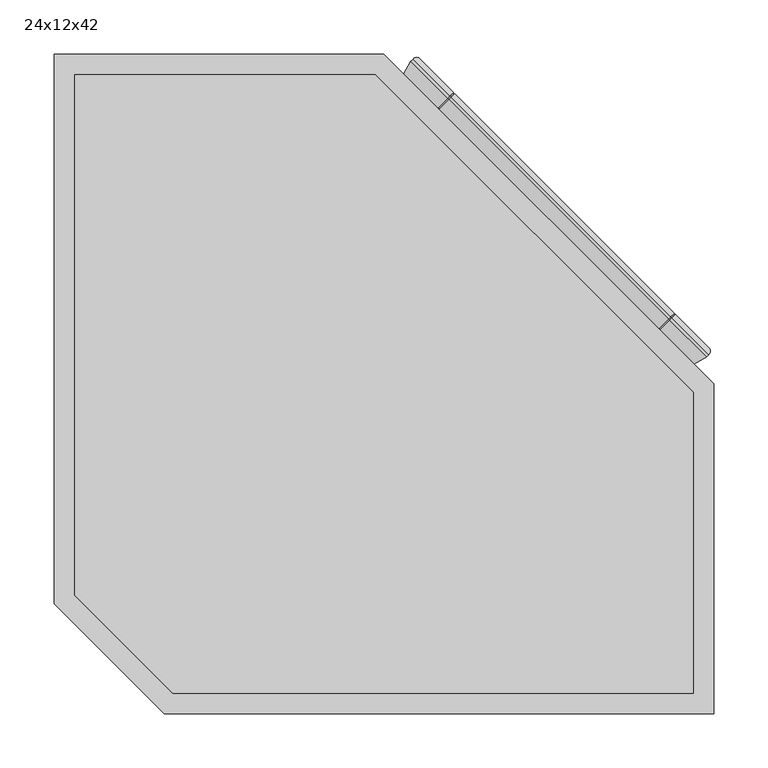
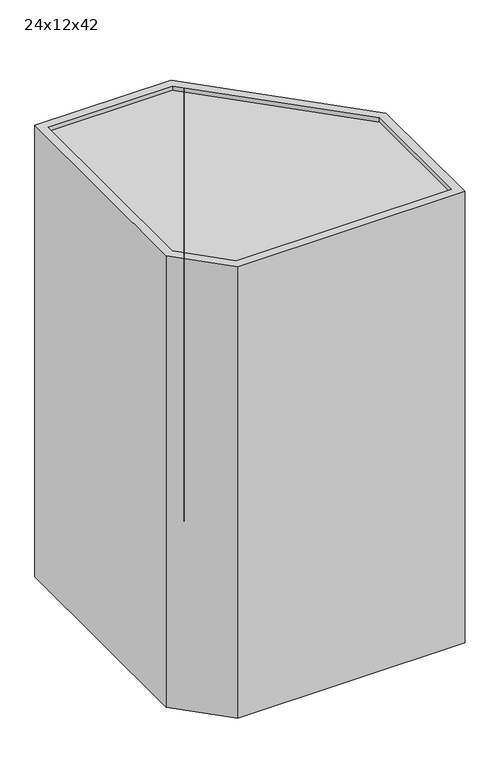
"""IFC4 building model written with IfcOpenShell, lengths in millimetres: furniture geometry, Cabinet-Wall-Merillat-Angle_Single_Door-Marlin : 24x12x42."""

from ifc_helpers import new_model, si_unit, frame, origin, place, context, project, spatial, polyline, circle_curve, ellipse_curve, outline, extrude, faceted_brep, source, transform, mapped, element, save
from ifc_brep_helpers import plane_surface, cylinder_surface, advanced_brep


def furniture_24x12x42_404ecca9(model_context):
    return source(origin(), model_context, "Body", "SolidModel", [
        advanced_brep(
        [(-277.8609132, 92.3131325, 2451.1), (-272.5103122, 93.2846318, 2448.0035075), (-272.5103122, 93.2846318, 1438.1964925), (-277.8609132, 92.3131325, 1435.1), (-279.818609, 90.3554366, 1435.1), (-279.818609, 90.3554366, 2451.1), (-286.5897222, 78.6272222, 1438.6052), (-286.5897222, 78.6272222, 2447.5948), (-254.9849038, 47.0224038, 2402.8988372), (-254.9849038, 47.0224038, 1483.3011628), (-254.1619151, 47.3219472, 1483.6712945), (-249.5344535, 49.0062055, 1485.7524535), (-249.5344535, 49.0062055, 2400.4475465), (-254.1619151, 47.3219472, 2402.5287055), (-248.9402505, 51.5799814, 1484.352684), (-248.9402505, 51.5799814, 2401.847316), (-258.8946123, 61.8880247, 1470.025), (-258.8946123, 61.8880247, 2416.175), (-255.4821149, 65.3005221, 1470.025), (-255.4821149, 65.3005221, 2416.175), (-245.1740716, 55.3461603, 1484.352684), (-245.1740716, 55.3461603, 2401.847316), (-242.6002957, 55.9403633, 1485.7524535), (-242.6002957, 55.9403633, 2400.4475465), (-240.9160374, 60.5678249, 1483.6712945), (-240.6188146, 61.3844378, 1483.3040302), (-240.616494, 61.3908136, 2402.8988372), (-240.9160374, 60.5678249, 2402.5287055), (-240.6144664, 61.388786, 1438.1964925), (-243.7755166, 58.2277358, 1435.1), (-3.5528682, -175.6728122, 1438.1964925), (-4.5243675, -181.0234132, 1435.1), (-38.5816131, -146.9661676, 1435.1), (-35.420563, -143.8051174, 1438.1964925), (-242.6529845, 57.1052038, 1435.1), (-239.4919344, 60.266254, 1438.1964925), (-36.543095, -142.6825854, 1438.1964925), (-39.7041452, -145.8436356, 1435.1), (-245.7332124, 56.27004, 1435.1), (-6.4820634, -182.981109, 1435.1), (-40.539309, -148.9238634, 1435.1), (-244.6106804, 55.147508, 1435.1), (-41.661841, -147.8013314, 1435.1), (-254.9828762, 47.0203762, 1438.6052), (-18.2102778, -189.7522222, 1438.6052), (-49.7889728, -158.1735272, 1438.6052), (-253.8603442, 45.8978442, 1438.6052), (-50.9115048, -157.0509952, 1438.6052), (-47.8312945, -152.6969535, 1485.7524535), (-253.2990782, 46.4591102, 1483.6712945), (-253.8603442, 45.8978442, 1483.3011628), (-50.9115048, -157.0509952, 1483.3011628), (-50.3502388, -156.4897292, 1483.6712945), (-49.5155528, -157.3244151, 1483.6712945), (-45.2575186, -152.1027505, 1484.352684), (-34.9494753, -162.0571123, 1470.025), (-31.5369779, -158.6446149, 1470.025), (-41.4913397, -148.3365716, 1484.352684), (-40.8971367, -145.7627957, 1485.7524535), (-36.2696751, -144.0785374, 1483.6712945), (-37.104361, -143.2438514, 1483.6712945), (-36.543095, -142.6825854, 1483.3011628), (-239.4919344, 60.266254, 1483.3011628), (-240.0532004, 59.704988, 1483.6712945), (-3.5528682, -175.6728122, 2448.0035075), (-4.5243675, -181.0234132, 2451.1), (-6.4820634, -182.981109, 2451.1), (-18.2102778, -189.7522222, 2447.5948), (-49.8150962, -158.1474038, 1483.3011628), (-49.8150962, -158.1474038, 2402.8988372), (-49.5155528, -157.3244151, 2402.5287055), (-47.8312945, -152.6969535, 2400.4475465), (-45.2575186, -152.1027505, 2401.847316), (-34.9494753, -162.0571123, 2416.175), (-31.5369779, -158.6446149, 2416.175), (-41.4913397, -148.3365716, 2401.847316), (-40.8971367, -145.7627957, 2400.4475465), (-36.2696751, -144.0785374, 2402.5287055), (-35.4466864, -143.778994, 2402.8988372), (-35.4466864, -143.778994, 1483.3011628), (-35.420563, -143.8051174, 2448.0035075), (-38.5816131, -146.9661676, 2451.1), (-243.7755166, 58.2277358, 2451.1), (-240.6144664, 61.388786, 2448.0035075), (-39.7041452, -145.8436356, 2451.1), (-36.543095, -142.6825854, 2448.0035075), (-239.4919344, 60.266254, 2448.0035075), (-242.6529845, 57.1052038, 2451.1), (-40.539309, -148.9238634, 2451.1), (-245.7332124, 56.27004, 2451.1), (-41.661841, -147.8013314, 2451.1), (-244.6106804, 55.147508, 2451.1), (-49.7889728, -158.1735272, 2447.5948), (-254.9828762, 47.0203762, 2447.5948), (-50.9115048, -157.0509952, 2447.5948), (-253.8603442, 45.8978442, 2447.5948), (-50.9115048, -157.0509952, 2402.8988372), (-253.8603442, 45.8978442, 2402.8988372), (-50.3502388, -156.4897292, 2402.5287055), (-253.2990782, 46.4591102, 2402.5287055), (-240.0532004, 59.704988, 2402.5287055), (-239.4919344, 60.266254, 2402.8988372), (-36.543095, -142.6825854, 2402.8988372), (-37.104361, -143.2438514, 2402.5287055), (-50.3502388, -156.4897292, 2446.9857412), (-41.5879457, -147.7274361, 2450.30625), (-39.7041452, -145.8436356, 2450.30625), (-37.104361, -143.2438514, 2447.8526052), (-35.981829, -144.3663834, 2402.5287055), (-35.981829, -144.3663834, 2447.8526052), (-38.5816131, -146.9661676, 2450.30625), (-40.4654137, -148.8499682, 2450.30625), (-49.2277068, -157.6122612, 2446.9857412), (-49.2277068, -157.6122612, 2402.5287055), (-254.4216102, 47.5816422, 2402.5287055), (-254.4216102, 47.5816422, 2446.9857412), (-245.6593171, 56.3439353, 2450.30625), (-243.7755166, 58.2277358, 2450.30625), (-241.1757324, 60.82752, 2447.8526052), (-241.1757324, 60.82752, 2402.5287055), (-240.0532004, 59.704988, 2447.8526052), (-242.6529845, 57.1052038, 2450.30625), (-244.5367851, 55.2214033, 2450.30625), (-253.2990782, 46.4591102, 2446.9857412), (-241.1757324, 60.82752, 1483.6712945), (-241.1757324, 60.82752, 1438.3473948), (-243.7755166, 58.2277358, 1435.89375), (-245.6593171, 56.3439353, 1435.89375), (-254.4216102, 47.5816422, 1439.2142588), (-254.4216102, 47.5816422, 1483.6712945), (-253.2990782, 46.4591102, 1439.2142588), (-244.5367851, 55.2214033, 1435.89375), (-242.6529845, 57.1052038, 1435.89375), (-240.0532004, 59.704988, 1438.3473948), (-37.104361, -143.2438514, 1438.3473948), (-39.7041452, -145.8436356, 1435.89375), (-41.5879457, -147.7274361, 1435.89375), (-50.3502388, -156.4897292, 1439.2142588), (-35.981829, -144.3663834, 1483.6712945), (-49.2277068, -157.6122612, 1483.6712945), (-49.2277068, -157.6122612, 1439.2142588), (-40.4654137, -148.8499682, 1435.89375), (-38.5816131, -146.9661676, 1435.89375), (-35.981829, -144.3663834, 1438.3473948)],
        [
            (0, 1, ellipse_curve(frame((-274.4843369, 88.9365562, 2446.3248), z_axis=(-0.5000000000000046, 0.49999999999999534, -0.7071067811865475), x_axis=(-0.5000000000000044, 0.4999999999999953, 0.7071067811865476)), 6.7531526, 4.7752)),
            (1, 2),
            (2, 3, ellipse_curve(frame((-274.4843369, 88.9365562, 1439.8752), z_axis=(-0.5000000000000046, 0.49999999999999534, 0.7071067811865475), x_axis=(0.5000000000000044, -0.4999999999999953, 0.7071067811865476)), 6.7531526, 4.7752)),
            (3, 0),
            (3, 4),
            (4, 5),
            (5, 0),
            (4, 6),
            (6, 7),
            (7, 5),
            (8, 9),
            (9, 10),
            (10, 11),
            (11, 12),
            (12, 13),
            (13, 8),
            (11, 14, ellipse_curve(frame((-250.0730668, 50.4860334, 1484.3252), z_axis=(-0.5000000000000047, 0.49999999999999545, 0.7071067811865475), x_axis=(0.5000000000000046, -0.49999999999999534, 0.7071067811865476)), 2.2271035, 1.5748)),
            (14, 15),
            (15, 12, ellipse_curve(frame((-250.0730668, 50.4860334, 2401.8748), z_axis=(-0.5000000000000047, 0.49999999999999545, -0.7071067811865475), x_axis=(-0.5000000000000046, 0.49999999999999534, 0.7071067811865476)), 2.2271035, 1.5748)),
            (14, 16),
            (16, 17),
            (17, 15),
            (16, 18),
            (18, 19),
            (19, 17),
            (18, 20),
            (20, 21),
            (21, 19),
            (20, 22, ellipse_curve(frame((-244.0801236, 56.4789766, 1484.3252), z_axis=(-0.5000000000000047, 0.49999999999999545, 0.7071067811865475), x_axis=(0.5000000000000046, -0.49999999999999534, 0.7071067811865476)), 2.2271035, 1.5748)),
            (22, 23),
            (23, 21, ellipse_curve(frame((-244.0801236, 56.4789766, 2401.8748), z_axis=(-0.5000000000000047, 0.49999999999999545, -0.7071067811865475), x_axis=(-0.5000000000000046, 0.49999999999999534, 0.7071067811865476)), 2.2271035, 1.5748)),
            (22, 24),
            (24, 25),
            (25, 26),
            (26, 27),
            (27, 23),
            (2, 28),
            (28, 29, circle_curve(frame((-243.7755166, 58.2277358, 1439.8752), z_axis=(-0.707106781186554, 0.707106781186541, 0.0), x_axis=(-0.707106781186541, -0.707106781186554, 0.0)), 4.7752)),
            (29, 3),
            (30, 31, ellipse_curve(frame((-7.9009438, -177.6468369, 1439.8752), z_axis=(-0.5000000000000046, 0.49999999999999534, -0.7071067811865475), x_axis=(-0.5000000000000047, 0.4999999999999955, 0.7071067811865475)), 6.7531526, 4.7752)),
            (31, 32),
            (32, 33, circle_curve(frame((-38.5816131, -146.9661676, 1439.8752), z_axis=(0.707106781186554, -0.707106781186541, 0.0), x_axis=(-0.707106781186541, -0.707106781186554, 0.0)), 4.7752)),
            (33, 30),
            (34, 35, circle_curve(frame((-242.6529845, 57.1052038, 1439.8752), z_axis=(0.707106781186554, -0.707106781186541, 0.0), x_axis=(-0.707106781186541, -0.707106781186554, 0.0)), 4.7752)),
            (35, 36),
            (36, 37, circle_curve(frame((-39.7041452, -145.8436356, 1439.8752), z_axis=(-0.707106781186554, 0.707106781186541, 0.0), x_axis=(-0.707106781186541, -0.707106781186554, 0.0)), 4.7752)),
            (37, 34),
            (29, 38),
            (38, 4),
            (31, 39),
            (39, 40),
            (40, 32),
            (41, 34),
            (37, 42),
            (42, 41),
            (38, 43),
            (43, 6),
            (39, 44),
            (44, 45),
            (45, 40),
            (46, 41),
            (42, 47),
            (47, 46),
            (48, 11),
            (10, 49),
            (49, 50),
            (50, 51),
            (51, 52),
            (52, 53),
            (53, 48),
            (48, 54, ellipse_curve(frame((-46.3514666, -153.2355668, 1484.3252), z_axis=(-0.5000000000000047, 0.49999999999999545, -0.7071067811865475), x_axis=(-0.5000000000000046, 0.49999999999999534, 0.7071067811865476)), 2.2271035, 1.5748)),
            (54, 14),
            (54, 55),
            (55, 16),
            (55, 56),
            (56, 18),
            (56, 57),
            (57, 20),
            (57, 58, ellipse_curve(frame((-40.3585234, -147.2426236, 1484.3252), z_axis=(-0.5000000000000047, 0.49999999999999545, -0.7071067811865475), x_axis=(-0.5000000000000046, 0.49999999999999534, 0.7071067811865476)), 2.2271035, 1.5748)),
            (58, 22),
            (58, 59),
            (59, 60),
            (60, 61),
            (61, 62),
            (62, 63),
            (63, 24),
            (30, 64),
            (64, 65, ellipse_curve(frame((-7.9009438, -177.6468369, 2446.3248), z_axis=(0.5000000000000046, -0.49999999999999534, -0.7071067811865475), x_axis=(-0.5000000000000044, 0.4999999999999953, -0.7071067811865476)), 6.7531526, 4.7752)),
            (65, 31),
            (65, 66),
            (66, 39),
            (66, 67),
            (67, 44),
            (68, 69),
            (69, 70),
            (70, 71),
            (71, 48),
            (53, 68),
            (71, 72, ellipse_curve(frame((-46.3514666, -153.2355668, 2401.8748), z_axis=(0.5000000000000047, -0.49999999999999545, -0.7071067811865475), x_axis=(-0.5000000000000046, 0.49999999999999534, -0.7071067811865476)), 2.2271035, 1.5748)),
            (72, 54),
            (72, 73),
            (73, 55),
            (73, 74),
            (74, 56),
            (74, 75),
            (75, 57),
            (75, 76, ellipse_curve(frame((-40.3585234, -147.2426236, 2401.8748), z_axis=(0.5000000000000047, -0.49999999999999545, -0.7071067811865475), x_axis=(-0.5000000000000046, 0.49999999999999534, -0.7071067811865476)), 2.2271035, 1.5748)),
            (76, 58),
            (76, 77),
            (77, 78),
            (78, 79),
            (79, 59),
            (64, 80),
            (80, 81, circle_curve(frame((-38.5816131, -146.9661676, 2446.3248), z_axis=(0.707106781186554, -0.707106781186541, 0.0), x_axis=(-0.707106781186541, -0.707106781186554, 0.0)), 4.7752)),
            (81, 65),
            (0, 82),
            (82, 83, circle_curve(frame((-243.7755166, 58.2277358, 2446.3248), z_axis=(-0.707106781186554, 0.707106781186541, 0.0), x_axis=(-0.707106781186541, -0.707106781186554, 0.0)), 4.7752)),
            (83, 1),
            (84, 85, circle_curve(frame((-39.7041452, -145.8436356, 2446.3248), z_axis=(-0.707106781186554, 0.707106781186541, 0.0), x_axis=(-0.707106781186541, -0.707106781186554, 0.0)), 4.7752)),
            (85, 86),
            (86, 87, circle_curve(frame((-242.6529845, 57.1052038, 2446.3248), z_axis=(0.707106781186554, -0.707106781186541, 0.0), x_axis=(-0.707106781186541, -0.707106781186554, 0.0)), 4.7752)),
            (87, 84),
            (81, 88),
            (88, 66),
            (5, 89),
            (89, 82),
            (90, 84),
            (87, 91),
            (91, 90),
            (88, 92),
            (92, 67),
            (7, 93),
            (93, 89),
            (94, 90),
            (91, 95),
            (95, 94),
            (43, 9),
            (8, 93),
            (92, 69),
            (68, 45),
            (96, 94),
            (95, 97),
            (97, 96),
            (50, 46),
            (47, 51),
            (12, 71),
            (70, 98),
            (98, 96),
            (97, 99),
            (99, 13),
            (15, 72),
            (17, 73),
            (19, 74),
            (21, 75),
            (23, 76),
            (27, 100),
            (100, 101),
            (101, 102),
            (102, 103),
            (103, 77),
            (83, 26),
            (25, 28),
            (33, 79),
            (78, 80),
            (85, 102),
            (101, 86),
            (35, 62),
            (61, 36),
            (98, 104),
            (104, 105),
            (105, 106),
            (106, 107, circle_curve(frame((-39.7041452, -145.8436356, 2446.3248), z_axis=(-0.7071067811865612, 0.7071067811865338, 0.0), x_axis=(0.0, 0.0, 1.0)), 3.98145)),
            (107, 103),
            (78, 108),
            (108, 109),
            (109, 110, circle_curve(frame((-38.5816131, -146.9661676, 2446.3248), z_axis=(0.7071067811865612, -0.7071067811865338, 0.0), x_axis=(0.0, 0.0, 1.0)), 3.98145)),
            (110, 111),
            (111, 112),
            (112, 113),
            (113, 69),
            (77, 108),
            (107, 109),
            (106, 110),
            (105, 111),
            (104, 112),
            (70, 113),
            (8, 114),
            (114, 115),
            (115, 116),
            (116, 117),
            (117, 118, circle_curve(frame((-243.7755166, 58.2277358, 2446.3248), z_axis=(-0.7071067811865612, 0.7071067811865338, 0.0), x_axis=(0.0, 0.0, 1.0)), 3.98145)),
            (118, 119),
            (119, 26),
            (100, 120),
            (120, 121, circle_curve(frame((-242.6529845, 57.1052038, 2446.3248), z_axis=(0.7071067811865612, -0.7071067811865338, 0.0), x_axis=(0.0, 0.0, 1.0)), 3.98145)),
            (121, 122),
            (122, 123),
            (123, 99),
            (119, 27),
            (118, 120),
            (117, 121),
            (116, 122),
            (115, 123),
            (114, 13),
            (25, 124),
            (124, 125),
            (125, 126, circle_curve(frame((-243.7755166, 58.2277358, 1439.8752), z_axis=(-0.7071067811865612, 0.7071067811865338, 0.0), x_axis=(0.0, 0.0, 1.0)), 3.98145)),
            (126, 127),
            (127, 128),
            (128, 129),
            (129, 9),
            (49, 130),
            (130, 131),
            (131, 132),
            (132, 133, circle_curve(frame((-242.6529845, 57.1052038, 1439.8752), z_axis=(0.7071067811865612, -0.7071067811865338, 0.0), x_axis=(0.0, 0.0, 1.0)), 3.98145)),
            (133, 63),
            (129, 10),
            (128, 130),
            (127, 131),
            (126, 132),
            (125, 133),
            (124, 24),
            (60, 134),
            (134, 135, circle_curve(frame((-39.7041452, -145.8436356, 1439.8752), z_axis=(-0.7071067811865612, 0.7071067811865338, 0.0), x_axis=(0.0, 0.0, 1.0)), 3.98145)),
            (135, 136),
            (136, 137),
            (137, 52),
            (138, 79),
            (68, 139),
            (139, 140),
            (140, 141),
            (141, 142),
            (142, 143, circle_curve(frame((-38.5816131, -146.9661676, 1439.8752), z_axis=(0.7071067811865612, -0.7071067811865338, 0.0), x_axis=(0.0, 0.0, 1.0)), 3.98145)),
            (143, 138),
            (138, 59),
            (53, 139),
            (137, 140),
            (136, 141),
            (135, 142),
            (134, 143),
        ],
        [
            cylinder_surface(frame((-274.4843369, 88.9365562, 2451.1), z_axis=(0.0, 0.0, 1.0), x_axis=(-0.7071067811865398, -0.7071067811865552, 0.0)), 4.7752),
            plane_surface(frame((-277.8609132, 92.3131325, 2451.1), z_axis=(-0.7071067811865552, 0.7071067811865398, 0.0), x_axis=(0.0, 0.0, -1.0))),
            plane_surface(frame((-279.818609, 90.3554366, 2451.1), z_axis=(-0.8660309890157606, 0.49999032597079685, 0.0), x_axis=(0.0, 0.0, -1.0))),
            plane_surface(frame((-254.9849038, 47.0224038, 2402.8988372), z_axis=(0.3420201433255881, -0.9396926207859378, 0.0), x_axis=(0.0, 0.0, -1.0))),
            cylinder_surface(frame((-250.0730668, 50.4860334, 2451.1), z_axis=(0.0, 0.0, 1.0000000000000002), x_axis=(0.7193398003386519, 0.6946583704589966, 0.0)), 1.5748),
            plane_surface(frame((-248.9402505, 51.5799814, 2401.847316), z_axis=(0.7193398003386716, 0.6946583704589762, 0.0), x_axis=(0.0, 0.0, -1.0))),
            plane_surface(frame((-258.8946123, 61.8880247, 2416.175), z_axis=(0.7071067811865552, -0.7071067811865398, 0.0), x_axis=(0.0, 0.0, -1.0))),
            plane_surface(frame((-255.4821149, 65.3005221, 2416.175), z_axis=(-0.6946583704589944, -0.7193398003386541, 0.0), x_axis=(0.0, 0.0, -1.0))),
            cylinder_surface(frame((-244.0801236, 56.4789766, 2451.1), z_axis=(0.0, 0.0, 1.0000000000000002), x_axis=(0.9396926207858448, -0.3420201433258438, 0.0)), 1.5748),
            plane_surface(frame((-242.6002957, 55.9403633, 2400.4475465), z_axis=(0.9396926207859251, -0.342020143325623, 0.0), x_axis=(0.0, 0.0, -1.0))),
            cylinder_surface(frame((-277.8609132, 92.3131325, 1439.8752), z_axis=(-0.707106781186554, 0.707106781186541, 0.0), x_axis=(-0.707106781186541, -0.707106781186554, 0.0)), 4.7752),
            plane_surface(frame((-277.8609132, 92.3131325, 1435.1), z_axis=(0.0, 0.0, -1.0), x_axis=(0.707106781186554, -0.707106781186541, 0.0))),
            plane_surface(frame((-279.818609, 90.3554366, 1435.1), z_axis=(-0.18302033152247393, -0.1830203315224773, -0.9659229350723619), x_axis=(0.707106781186554, -0.707106781186541, 0.0))),
            plane_surface(frame((-254.9849038, 47.0224038, 1483.3011628), z_axis=(-0.298836238730178, -0.2988362387301835, 0.9063077870366099), x_axis=(0.707106781186554, -0.707106781186541, 0.0))),
            cylinder_surface(frame((-284.8805396, 85.2935061, 1484.3252), z_axis=(-0.7071067811865541, 0.7071067811865411, 0.0), x_axis=(0.7069990853988176, 0.7069990853988306, 0.01745240643729364)), 1.5748),
            plane_surface(frame((-248.9402505, 51.5799814, 1484.352684), z_axis=(0.7069990853988173, 0.7069990853988303, 0.017452406437322147), x_axis=(0.707106781186554, -0.707106781186541, 0.0))),
            plane_surface(frame((-258.8946123, 61.8880247, 1470.025), z_axis=(0.0, 0.0, 1.0), x_axis=(0.707106781186554, -0.707106781186541, 0.0))),
            plane_surface(frame((-255.4821149, 65.3005221, 1470.025), z_axis=(-0.7069990853988178, -0.7069990853988308, 0.01745240643727848), x_axis=(0.707106781186554, -0.707106781186541, 0.0))),
            cylinder_surface(frame((-278.8875963, 91.2864494, 1484.3252), z_axis=(-0.7071067811865541, 0.7071067811865411, 0.0), x_axis=(0.2988362387299919, 0.29883623872999737, 0.9063077870367326)), 1.5748),
            plane_surface(frame((-242.6002957, 55.9403633, 1485.7524535), z_axis=(0.29883623873014237, 0.29883623873014786, 0.9063077870366333), x_axis=(0.707106781186554, -0.707106781186541, 0.0))),
            cylinder_surface(frame((-7.9009438, -177.6468369, 1435.1), z_axis=(0.0, 0.0, -1.0), x_axis=(-0.7071067811865422, -0.7071067811865528, 0.0)), 4.7752),
            plane_surface(frame((-4.5243675, -181.0234132, 1435.1), z_axis=(0.7071067811865528, -0.7071067811865422, 0.0), x_axis=(0.0, 0.0, 1.0))),
            plane_surface(frame((-6.4820634, -182.981109, 1435.1), z_axis=(0.4999903259708127, -0.8660309890157514, 0.0), x_axis=(0.0, 0.0, 1.0))),
            plane_surface(frame((-49.8150962, -158.1474038, 1483.3011628), z_axis=(-0.939692620785944, 0.3420201433255708, 0.0), x_axis=(0.0, 0.0, 1.0))),
            cylinder_surface(frame((-46.3514666, -153.2355668, 1435.1), z_axis=(0.0, 0.0, -1.0000000000000002), x_axis=(0.6946583704589834, 0.7193398003386646, 0.0)), 1.5748),
            plane_surface(frame((-45.2575186, -152.1027505, 1484.352684), z_axis=(0.694658370458963, 0.7193398003386844, 0.0), x_axis=(0.0, 0.0, 1.0))),
            plane_surface(frame((-34.9494753, -162.0571123, 1470.025), z_axis=(-0.7071067811865528, 0.7071067811865422, 0.0), x_axis=(0.0, 0.0, 1.0))),
            plane_surface(frame((-31.5369779, -158.6446149, 1470.025), z_axis=(-0.7193398003386413, -0.6946583704590076, 0.0), x_axis=(0.0, 0.0, 1.0))),
            cylinder_surface(frame((-40.3585234, -147.2426236, 1435.1), z_axis=(0.0, 0.0, -1.0000000000000002), x_axis=(-0.34202014332586106, 0.9396926207858385, 0.0)), 1.5748),
            plane_surface(frame((-40.8971367, -145.7627957, 1485.7524535), z_axis=(-0.3420201433256403, 0.9396926207859188, 0.0), x_axis=(0.0, 0.0, 1.0))),
            cylinder_surface(frame((-4.5243675, -181.0234132, 2446.3248), z_axis=(0.707106781186554, -0.707106781186541, 0.0), x_axis=(-0.707106781186541, -0.707106781186554, 0.0)), 4.7752),
            plane_surface(frame((-4.5243675, -181.0234132, 2451.1), z_axis=(0.0, 0.0, 1.0), x_axis=(-0.707106781186554, 0.707106781186541, 0.0))),
            plane_surface(frame((-6.4820634, -182.981109, 2451.1), z_axis=(-0.18302033152247393, -0.1830203315224773, 0.9659229350723619), x_axis=(-0.707106781186554, 0.707106781186541, 0.0))),
            plane_surface(frame((-18.2102778, -189.7522222, 2447.5948), z_axis=(-0.707106781186541, -0.707106781186554, 0.0), x_axis=(-0.707106781186554, 0.707106781186541, 0.0))),
            plane_surface(frame((-49.8150962, -158.1474038, 2402.8988372), z_axis=(-0.298836238730178, -0.2988362387301835, -0.9063077870366099), x_axis=(-0.707106781186554, 0.707106781186541, 0.0))),
            cylinder_surface(frame((-11.5439939, -188.0430396, 2401.8748), z_axis=(0.7071067811865541, -0.7071067811865411, 0.0), x_axis=(0.7069990853988176, 0.7069990853988306, -0.01745240643729364)), 1.5748),
            plane_surface(frame((-45.2575186, -152.1027505, 2401.847316), z_axis=(0.7069990853988173, 0.7069990853988303, -0.017452406437322147), x_axis=(-0.707106781186554, 0.707106781186541, 0.0))),
            plane_surface(frame((-34.9494753, -162.0571123, 2416.175), z_axis=(0.0, 0.0, -1.0), x_axis=(-0.707106781186554, 0.707106781186541, 0.0))),
            plane_surface(frame((-31.5369779, -158.6446149, 2416.175), z_axis=(-0.7069990853988178, -0.7069990853988308, -0.01745240643727848), x_axis=(-0.707106781186554, 0.707106781186541, 0.0))),
            cylinder_surface(frame((-5.5510506, -182.0500963, 2401.8748), z_axis=(0.7071067811865541, -0.7071067811865411, 0.0), x_axis=(0.2988362387299919, 0.29883623872999737, -0.9063077870367326)), 1.5748),
            plane_surface(frame((-40.8971367, -145.7627957, 2400.4475465), z_axis=(0.29883623873014237, 0.29883623873014786, -0.9063077870366333), x_axis=(-0.707106781186554, 0.707106781186541, 0.0))),
            plane_surface(frame((-35.4466864, -143.778994, 2402.8988372), z_axis=(0.707106781186541, 0.707106781186554, 0.0), x_axis=(-0.707106781186554, 0.707106781186541, 0.0))),
            plane_surface(frame((-36.543095, -142.6825854, 2402.8988372), z_axis=(0.7071067811865612, -0.7071067811865337, 0.0), x_axis=(-0.6408563820557478, -0.6408563820557727, -0.4226182617407854))),
            plane_surface(frame((-35.420563, -143.8051174, 2402.8988372), z_axis=(-0.7071067811865612, 0.7071067811865337, 0.0), x_axis=(0.6408563820557478, 0.6408563820557727, 0.4226182617407854))),
            plane_surface(frame((-36.543095, -142.6825854, 2402.8988372), z_axis=(-0.2988362387301747, -0.2988362387301865, 0.9063077870366099), x_axis=(0.7071067811865616, -0.7071067811865335, 0.0))),
            plane_surface(frame((-37.104361, -143.2438514, 2402.5287055), z_axis=(0.7071067811865335, 0.7071067811865616, 0.0), x_axis=(0.7071067811865616, -0.7071067811865335, 0.0))),
            cylinder_surface(frame((-38.5816131, -146.9661676, 2446.3248), z_axis=(0.7071067811865612, -0.7071067811865338, 0.0), x_axis=(0.0, 0.0, 1.0)), 3.98145),
            plane_surface(frame((-39.7041452, -145.8436356, 2450.30625), z_axis=(0.0, 0.0, 1.0), x_axis=(0.7071067811865616, -0.7071067811865335, 0.0))),
            plane_surface(frame((-41.5879457, -147.7274361, 2450.30625), z_axis=(-0.18302033152251398, -0.18302033152252126, 0.965922935072346), x_axis=(0.7071067811865616, -0.7071067811865335, 0.0))),
            plane_surface(frame((-50.3502388, -156.4897292, 2446.9857412), z_axis=(-0.7071067811865335, -0.7071067811865616, 0.0), x_axis=(0.7071067811865616, -0.7071067811865335, 0.0))),
            plane_surface(frame((-50.3502388, -156.4897292, 2402.5287055), z_axis=(0.29883623873019277, 0.2988362387302046, 0.906307787036598), x_axis=(0.7071067811865616, -0.7071067811865335, 0.0))),
            plane_surface(frame((-240.6144664, 61.388786, 2402.8988372), z_axis=(0.7071067811865612, -0.7071067811865337, 0.0), x_axis=(-0.6408563820557478, -0.6408563820557727, -0.4226182617407854))),
            plane_surface(frame((-239.4919344, 60.266254, 2402.8988372), z_axis=(-0.7071067811865612, 0.7071067811865337, 0.0), x_axis=(0.6408563820557478, 0.6408563820557727, 0.4226182617407854))),
            plane_surface(frame((-240.6144664, 61.388786, 2402.8988372), z_axis=(-0.2988362387301747, -0.2988362387301865, 0.9063077870366099), x_axis=(0.7071067811865616, -0.7071067811865335, 0.0))),
            plane_surface(frame((-241.1757324, 60.82752, 2402.5287055), z_axis=(0.7071067811865335, 0.7071067811865616, 0.0), x_axis=(0.7071067811865616, -0.7071067811865335, 0.0))),
            cylinder_surface(frame((-242.6529845, 57.1052038, 2446.3248), z_axis=(0.7071067811865612, -0.7071067811865338, 0.0), x_axis=(0.0, 0.0, 1.0)), 3.98145),
            plane_surface(frame((-243.7755166, 58.2277358, 2450.30625), z_axis=(0.0, 0.0, 1.0), x_axis=(0.7071067811865616, -0.7071067811865335, 0.0))),
            plane_surface(frame((-245.6593171, 56.3439353, 2450.30625), z_axis=(-0.18302033152251576, -0.18302033152252303, 0.9659229350723454), x_axis=(0.7071067811865616, -0.7071067811865335, 0.0))),
            plane_surface(frame((-254.4216102, 47.5816422, 2446.9857412), z_axis=(-0.7071067811865354, -0.7071067811865597, 0.0), x_axis=(0.7071067811865597, -0.7071067811865354, 0.0))),
            plane_surface(frame((-254.4216102, 47.5816422, 2402.5287055), z_axis=(0.29883623873019416, 0.29883623873020443, 0.9063077870365974), x_axis=(0.7071067811865597, -0.7071067811865354, 0.0))),
            plane_surface(frame((-243.7755166, 58.2277358, 1444.6504), z_axis=(0.7071067811865612, -0.7071067811865338, 0.0), x_axis=(0.7071067811865338, 0.7071067811865612, 0.0))),
            plane_surface(frame((-242.6529845, 57.1052038, 1444.6504), z_axis=(-0.7071067811865612, 0.7071067811865338, 0.0), x_axis=(-0.7071067811865338, -0.7071067811865612, 0.0))),
            plane_surface(frame((-254.9828762, 47.0203762, 1483.3011628), z_axis=(0.2988362387301807, 0.2988362387301926, -0.906307787036606), x_axis=(0.7071067811865616, -0.7071067811865335, 0.0))),
            plane_surface(frame((-254.4216102, 47.5816422, 1483.6712945), z_axis=(-0.7071067811865335, -0.7071067811865616, 0.0), x_axis=(0.7071067811865616, -0.7071067811865335, 0.0))),
            plane_surface(frame((-254.4216102, 47.5816422, 1439.2142588), z_axis=(-0.18302033152271646, -0.18302033152272373, -0.9659229350722693), x_axis=(0.7071067811865616, -0.7071067811865335, 0.0))),
            plane_surface(frame((-245.6593171, 56.3439353, 1435.89375), z_axis=(0.0, 0.0, -1.0), x_axis=(0.7071067811865616, -0.7071067811865335, 0.0))),
            cylinder_surface(frame((-242.6529845, 57.1052038, 1439.8752), z_axis=(0.7071067811865612, -0.7071067811865338, 0.0), x_axis=(0.0, 0.0, 1.0)), 3.98145),
            plane_surface(frame((-241.1757324, 60.82752, 1438.3473948), z_axis=(0.7071067811865335, 0.7071067811865616, 0.0), x_axis=(0.7071067811865616, -0.7071067811865335, 0.0))),
            plane_surface(frame((-241.1757324, 60.82752, 1483.6712945), z_axis=(-0.29883623873017934, -0.2988362387301912, -0.906307787036607), x_axis=(0.7071067811865616, -0.7071067811865335, 0.0))),
            plane_surface(frame((-37.104361, -143.2438514, 1483.6712945), z_axis=(0.7071067811865613, -0.7071067811865339, 0.0), x_axis=(0.6408563820557613, 0.6408563820557862, -0.42261826174074446))),
            plane_surface(frame((-35.981829, -144.3663834, 1483.6712945), z_axis=(-0.7071067811865613, 0.7071067811865339, 0.0), x_axis=(-0.6408563820557613, -0.6408563820557862, 0.42261826174074446))),
            plane_surface(frame((-37.104361, -143.2438514, 1483.6712945), z_axis=(-0.2988362387301457, -0.2988362387301576, -0.9063077870366291), x_axis=(0.7071067811865616, -0.7071067811865335, 0.0))),
            plane_surface(frame((-50.9115048, -157.0509952, 1483.3011628), z_axis=(0.2988362387301807, 0.2988362387301926, -0.906307787036606), x_axis=(0.7071067811865616, -0.7071067811865335, 0.0))),
            plane_surface(frame((-50.3502388, -156.4897292, 1483.6712945), z_axis=(-0.7071067811865335, -0.7071067811865616, 0.0), x_axis=(0.7071067811865616, -0.7071067811865335, 0.0))),
            plane_surface(frame((-50.3502388, -156.4897292, 1439.2142588), z_axis=(-0.1830203315227165, -0.18302033152272376, -0.9659229350722693), x_axis=(0.7071067811865616, -0.7071067811865335, 0.0))),
            plane_surface(frame((-41.5879457, -147.7274361, 1435.89375), z_axis=(0.0, 0.0, -1.0), x_axis=(0.7071067811865616, -0.7071067811865335, 0.0))),
            cylinder_surface(frame((-38.5816131, -146.9661676, 1439.8752), z_axis=(0.7071067811865612, -0.7071067811865338, 0.0), x_axis=(0.0, 0.0, 1.0)), 3.98145),
            plane_surface(frame((-37.104361, -143.2438514, 1438.3473948), z_axis=(0.7071067811865335, 0.7071067811865616, 0.0), x_axis=(0.7071067811865616, -0.7071067811865335, 0.0))),
        ],
        [
            (0, [[1, 2, 3, 4]]),
            (1, [[-4, 5, 6, 7]]),
            (2, [[-6, 8, 9, 10]]),
            (3, [[11, 12, 13, 14, 15, 16]]),
            (4, [[-14, 17, 18, 19]]),
            (5, [[-18, 20, 21, 22]]),
            (6, [[-21, 23, 24, 25]]),
            (7, [[-24, 26, 27, 28]]),
            (8, [[-27, 29, 30, 31]]),
            (9, [[-30, 32, 33, 34, 35, 36]]),
            (10, [[-3, 37, 38, 39]]),
            (10, [[40, 41, 42, 43]]),
            (10, [[44, 45, 46, 47]]),
            (11, [[-5, -39, 48, 49]]),
            (11, [[50, 51, 52, -41]]),
            (11, [[53, -47, 54, 55]]),
            (12, [[-8, -49, 56, 57]]),
            (12, [[58, 59, 60, -51]]),
            (12, [[61, -55, 62, 63]]),
            (13, [[64, -13, 65, 66, 67, 68, 69, 70]]),
            (14, [[-17, -64, 71, 72]]),
            (15, [[-20, -72, 73, 74]]),
            (16, [[-23, -74, 75, 76]]),
            (17, [[-26, -76, 77, 78]]),
            (18, [[-29, -78, 79, 80]]),
            (19, [[-80, 81, 82, 83, 84, 85, 86, -32]]),
            (20, [[-40, 87, 88, 89]]),
            (21, [[-50, -89, 90, 91]]),
            (22, [[-58, -91, 92, 93]]),
            (23, [[94, 95, 96, 97, -70, 98]]),
            (24, [[-71, -97, 99, 100]]),
            (25, [[-73, -100, 101, 102]]),
            (26, [[-75, -102, 103, 104]]),
            (27, [[-77, -104, 105, 106]]),
            (28, [[-79, -106, 107, 108]]),
            (29, [[-108, 109, 110, 111, 112, -81]]),
            (30, [[-88, 113, 114, 115]]),
            (30, [[-1, 116, 117, 118]]),
            (30, [[119, 120, 121, 122]]),
            (31, [[-90, -115, 123, 124]]),
            (31, [[-7, 125, 126, -116]]),
            (31, [[127, -122, 128, 129]]),
            (32, [[-92, -124, 130, 131]]),
            (32, [[-10, 132, 133, -125]]),
            (32, [[134, -129, 135, 136]]),
            (33, [[-9, -57, 137, -11, 138, -132]]),
            (33, [[-93, -131, 139, -94, 140, -59]]),
            (33, [[141, -136, 142, 143]]),
            (33, [[144, -63, 145, -67]]),
            (34, [[146, -96, 147, 148, -143, 149, 150, -15]]),
            (35, [[-19, 151, -99, -146]]),
            (36, [[-22, 152, -101, -151]]),
            (37, [[-25, 153, -103, -152]]),
            (38, [[-28, 154, -105, -153]]),
            (39, [[-31, 155, -107, -154]]),
            (40, [[-155, -36, 156, 157, 158, 159, 160, -109]]),
            (41, [[-2, -118, 161, -34, 162, -37]]),
            (41, [[-87, -43, 163, -111, 164, -113]]),
            (41, [[165, -158, 166, -120]]),
            (41, [[167, -84, 168, -45]]),
            (42, [[169, 170, 171, 172, 173, -159, -165, -119, -127, -134, -141, -148]]),
            (43, [[174, 175, 176, 177, 178, 179, 180, -139, -130, -123, -114, -164]]),
            (44, [[-174, -110, 181]]),
            (45, [[-173, 182, -175, -181, -160]]),
            (46, [[-172, 183, -176, -182]]),
            (47, [[-171, 184, -177, -183]]),
            (48, [[-170, 185, -178, -184]]),
            (49, [[-169, -147, 186, -179, -185]]),
            (50, [[-180, -186, -95]]),
            (51, [[187, 188, 189, 190, 191, 192, 193, -161, -117, -126, -133, -138]]),
            (52, [[194, 195, 196, 197, 198, -149, -142, -135, -128, -121, -166, -157]]),
            (53, [[-193, 199, -35]]),
            (54, [[-192, 200, -194, -156, -199]]),
            (55, [[-191, 201, -195, -200]]),
            (56, [[-190, 202, -196, -201]]),
            (57, [[-189, 203, -197, -202]]),
            (58, [[-188, 204, -150, -198, -203]]),
            (59, [[-187, -16, -204]]),
            (60, [[205, 206, 207, 208, 209, 210, 211, -137, -56, -48, -38, -162]]),
            (61, [[212, 213, 214, 215, 216, -85, -167, -44, -53, -61, -144, -66]]),
            (62, [[-211, 217, -12]]),
            (63, [[-210, 218, -212, -65, -217]]),
            (64, [[-209, 219, -213, -218]]),
            (65, [[-208, 220, -214, -219]]),
            (66, [[-207, 221, -215, -220]]),
            (67, [[-206, 222, -86, -216, -221]]),
            (68, [[-205, -33, -222]]),
            (69, [[223, 224, 225, 226, 227, -68, -145, -62, -54, -46, -168, -83]]),
            (70, [[228, -163, -42, -52, -60, -140, 229, 230, 231, 232, 233, 234]]),
            (71, [[-228, 235, -112]]),
            (72, [[-229, -98, 236]]),
            (73, [[-227, 237, -230, -236, -69]]),
            (74, [[-226, 238, -231, -237]]),
            (75, [[-225, 239, -232, -238]]),
            (76, [[-224, 240, -233, -239]]),
            (77, [[-223, -82, -235, -234, -240]]),
        ],
    ),
        extrude(outline(polyline([(-31.5369779, -158.6446149), (-34.9494753, -162.0571123), (-258.8946123, 61.8880247), (-255.4821149, 65.3005221), (-31.5369779, -158.6446149)])), frame((0.0, 0.0, 1470.025), z_axis=(0.0, 0.0, 1.0), x_axis=(1.0, 0.0, 0.0)), (0.0, 0.0, 1.0), 946.15),
        faceted_brep([(-296.0453842, 61.1421158, 2438.4), (-282.575, 74.6125, 2438.4), (-22.225, -185.7375, 2438.4), (-35.6953842, -199.2078842, 2438.4), (-35.6953842, -199.2078842, 1447.8), (-22.225, -185.7375, 1447.8), (-282.575, 74.6125, 1447.8), (-296.0453842, 61.1421158, 1447.8), (-609.6, 96.8375, 2476.5), (-609.6, -411.1625, 2476.5), (-508.0, -512.7625, 2476.5), (0.0, -512.7625, 2476.5), (0.0, -207.9625, 2476.5), (-304.8, 96.8375, 2476.5), (-19.05, -215.8532684, 2476.5), (-19.05, -493.7125, 2476.5), (-500.1092316, -493.7125, 2476.5), (-590.55, -403.2717316, 2476.5), (-590.55, 77.7875, 2476.5), (-312.6907684, 77.7875, 2476.5), (-609.6, 96.8375, 1409.7), (-304.8, 96.8375, 1409.7), (0.0, -207.9625, 1409.7), (0.0, -512.7625, 1409.7), (-508.0, -512.7625, 1409.7), (-609.6, -411.1625, 1409.7), (-19.05, -215.8532684, 1409.7), (-312.6907684, 77.7875, 1409.7), (-590.55, 77.7875, 1409.7), (-590.55, -403.2717316, 1409.7), (-500.1092316, -493.7125, 1409.7), (-19.05, -493.7125, 1409.7)], [[[0, 1, 2, 3]], [[4, 5, 6, 7]], [[3, 2, 5, 4]], [[1, 0, 7, 6]], [[8, 9, 10, 11, 12, 13], [14, 15, 16, 17, 18, 19]], [[20, 21, 22, 23, 24, 25], [26, 27, 28, 29, 30, 31]], [[9, 8, 20, 25]], [[10, 9, 25, 24]], [[11, 10, 24, 23]], [[12, 11, 23, 22]], [[13, 12, 22, 21], [2, 1, 6, 5]], [[8, 13, 21, 20]], [[15, 14, 26, 31]], [[16, 15, 31, 30]], [[17, 16, 30, 29]], [[18, 17, 29, 28]], [[19, 18, 28, 27]], [[14, 19, 27, 26], [0, 3, 4, 7]]]),
        extrude(outline(polyline([(-312.6907684, 77.7875), (-19.05, -215.8532684), (-19.05, -493.7125), (-500.1092316, -493.7125), (-590.55, -403.2717316), (-590.55, 77.7875), (-312.6907684, 77.7875)])), frame((0.0, 0.0, 2200.275), z_axis=(0.0, 0.0, 1.0), x_axis=(1.0, 0.0, 0.0)), (0.0, 0.0, 1.0), 19.05),
        extrude(outline(polyline([(-312.6907684, 77.7875), (-19.05, -215.8532684), (-19.05, -493.7125), (-500.1092316, -493.7125), (-590.55, -403.2717316), (-590.55, 77.7875), (-312.6907684, 77.7875)])), frame((0.0, 0.0, 1933.575), z_axis=(0.0, 0.0, 1.0), x_axis=(1.0, 0.0, 0.0)), (0.0, 0.0, 1.0), 19.05),
        extrude(outline(polyline([(-312.6907684, 77.7875), (-19.05, -215.8532684), (-19.05, -493.7125), (-500.1092316, -493.7125), (-590.55, -403.2717316), (-590.55, 77.7875), (-312.6907684, 77.7875)])), frame((0.0, 0.0, 1666.875), z_axis=(0.0, 0.0, 1.0), x_axis=(1.0, 0.0, 0.0)), (0.0, 0.0, 1.0), 19.05),
        extrude(outline(polyline([(-590.55, -403.2717316), (-590.55, 77.7875), (-312.6907684, 77.7875), (-19.05, -215.8532684), (-19.05, -493.7125), (-500.1092316, -493.7125), (-590.55, -403.2717316)])), frame((0.0, 0.0, 2447.925), z_axis=(0.0, 0.0, 1.0), x_axis=(1.0, 0.0, 0.0)), (0.0, 0.0, 1.0), 19.05),
        extrude(outline(polyline([(-312.6907684, 77.7875), (-19.05, -215.8532684), (-19.05, -493.7125), (-500.1092316, -493.7125), (-590.55, -403.2717316), (-590.55, 77.7875), (-312.6907684, 77.7875)])), frame((0.0, 0.0, 1419.225), z_axis=(0.0, 0.0, 1.0), x_axis=(1.0, 0.0, 0.0)), (0.0, 0.0, 1.0), 19.05),
    ])


if __name__ == "__main__":
    model = new_model("IFC4")
    model_context = context("Model", 3, world=origin())
    ifc_project = project(units=[si_unit("LENGTHUNIT", "METRE", prefix="MILLI")], contexts=[model_context])
    site = spatial("IfcSite", under=ifc_project)
    building = spatial("IfcBuilding", under=site)
    placement = place(None, origin())
    furniture_24x12x42_shape = furniture_24x12x42_404ecca9(model_context)
    element("IfcFurniture", 1, ObjectType="Cabinet-Wall-Merillat-Angle_Single_Door-Marlin : 24x12x42", at=placement, inside=building, context=model_context, shape_type="MappedRepresentation", body=[
        mapped(furniture_24x12x42_shape, transform((0.0, 0.0, 0.0), x_axis=(1.0, 0.0, 0.0), y_axis=(0.0, 1.0, 0.0), z_axis=(0.0, 0.0, 1.0))),
    ])
    save(model, "model.ifc")

# Revit data of these elements
# Type "Cabinet-Wall-Merillat-Angle_Single_Door-Marlin : 24x12x42"
#   URL = "http://www.merillat.com/"
#   Product Page URL = "http://www.merillat.com/our-products/"
#   Product Line = "\"Express\""
#   Product Group = "Wall Cabinet"
#   Product Documentation Link = "http://merillatbusiness.com/wp-content/uploads/2014/07/Merillat_Classic_Catalog.pdf"
#   Model = "WA2442 R or L"
#   Manufacturer = "Merillat"
#   Glass Door Note = "Glass Cabinet doors are only available in specific sizes. Please refer to the catalog for this information before requesting a glass size"
#   Finish = "Wood"
#   Description = "Wall Angle Single Door Cabinet"
#   Construction Type = "Wall Angle Cabinet"
#   Cabinet Construction Note = "Requires 24  1/16 inches of wall space excluding dining room side cabinet door"
#   Assembly Code = "C1030410"
#   Width = 2' - 0"
#   Top of Cabinet = 8' - 0"
#   Spacing = 0' - 1"
#   Shelving Height = 0' - 10 1/2"
#   Height = 3' - 6"
#   Door Spacing = 0' - 1 3/4"
#   Depth = 1' - 0"
#   Cabinet Shell = 0' - 0 3/4"
#   Cabinet Door Width = 1' - 3 7/32"
#   Cabinet Door Height = 3' - 4"
#   COBie.Type = no
#   Solid Panel Door = no
#   Partial Overlay = yes
#   Number of Shelves = 3
#   Middle Shelf = yes
#   Glass Door = yes
#   Full Overlay = no
#   Elevation Swing Line = yes
#   Door Drawer Material = Wood - Merillat - Pecan(1)
#   Cabinet Material = Wood - Merillat - Pecan(1)
# Element 1 (IfcFurniture, "Cabinet-Wall-Merillat-Angle_Single_Door-Marlin : 24x12x42")
#   Materials on its faces: "Wood - Merillat - Pecan(1)"
# Materials
#   "Wood - Merillat - Pecan(1)": class "Wood", colour RGB 108 67 43, transparency 0, Cost = 0
